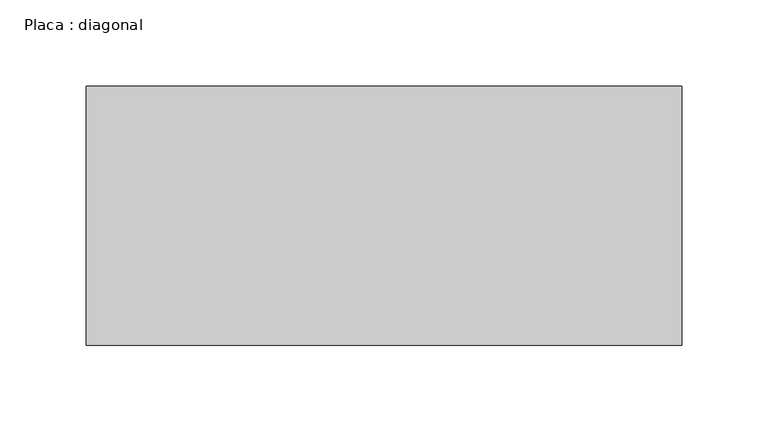
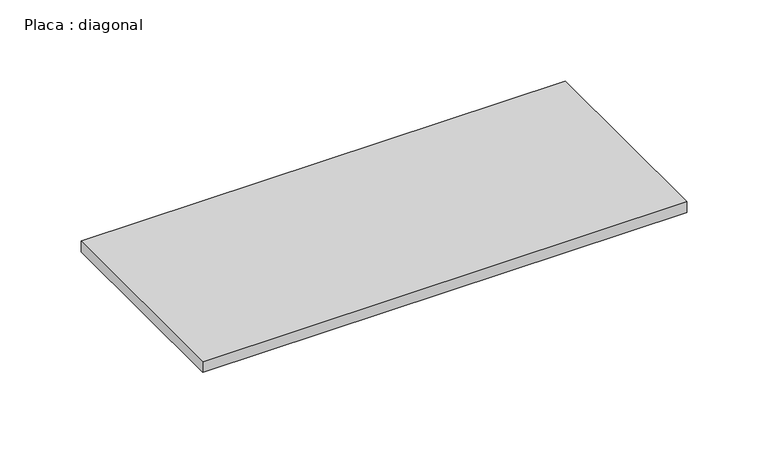
"""IFC4 building model written with IfcOpenShell, lengths in millimetres: beam geometry, Placa : diagonal."""

from ifc_helpers import new_model, si_unit, frame, origin, place, context, project, spatial, polyline, outline, extrude, source, transform, mapped, element, save


def placa_diagonal_616b5fb7(model_context):
    return source(origin(), model_context, "Body", "SweptSolid", [
        extrude(outline(polyline([(172.7806227, 75.0), (172.7806227, -75.0), (-171.8235671, -75.0), (-171.8235671, 75.0), (172.7806227, 75.0)])), frame((0.0, 0.0, -4.0), z_axis=(0.0, 0.0, 1.0), x_axis=(1.0, 0.0, 0.0)), (0.0, 0.0, 1.0), 8.0),
    ])


if __name__ == "__main__":
    model = new_model("IFC4")
    model_context = context("Model", 3, world=origin())
    ifc_project = project(units=[si_unit("LENGTHUNIT", "METRE", prefix="MILLI")], contexts=[model_context])
    site = spatial("IfcSite", under=ifc_project)
    building = spatial("IfcBuilding", under=site)
    placement = place(None, origin())
    placa_diagonal_shape = placa_diagonal_616b5fb7(model_context)
    element("IfcBeam", 1, ObjectType="Placa : diagonal", at=placement, inside=building, context=model_context, shape_type="MappedRepresentation", body=[
        mapped(placa_diagonal_shape, transform((0.0, 0.0, 0.0), x_axis=(1.0, 0.0, 0.0), y_axis=(0.0, 1.0, 0.0), z_axis=(0.0, 0.0, 1.0))),
    ])
    save(model, "model.ifc")

# Revit data of these elements
# Type "Placa : diagonal"
#   W = 0
#   Length [instance default] = 1.50 m
#   b = 0.15 m
#   d = 0.008 m
#   A = 0 m²
#   Structural Material [instance default] = Aço, 45-345
# Element 1 (IfcBeam, "Placa : diagonal")
#   Materials on its faces: "Aço, 45-345"
# Materials
#   "Aço, 45-345": class "Metal", colour RGB 247 247 247, transparency 0, Description = "Aço 345 MPa", Cost = 0
